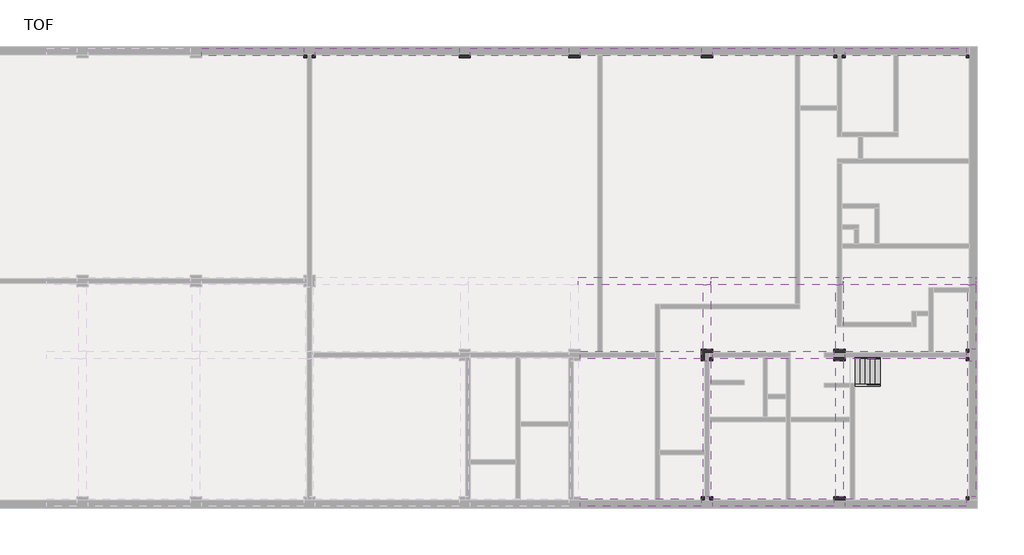
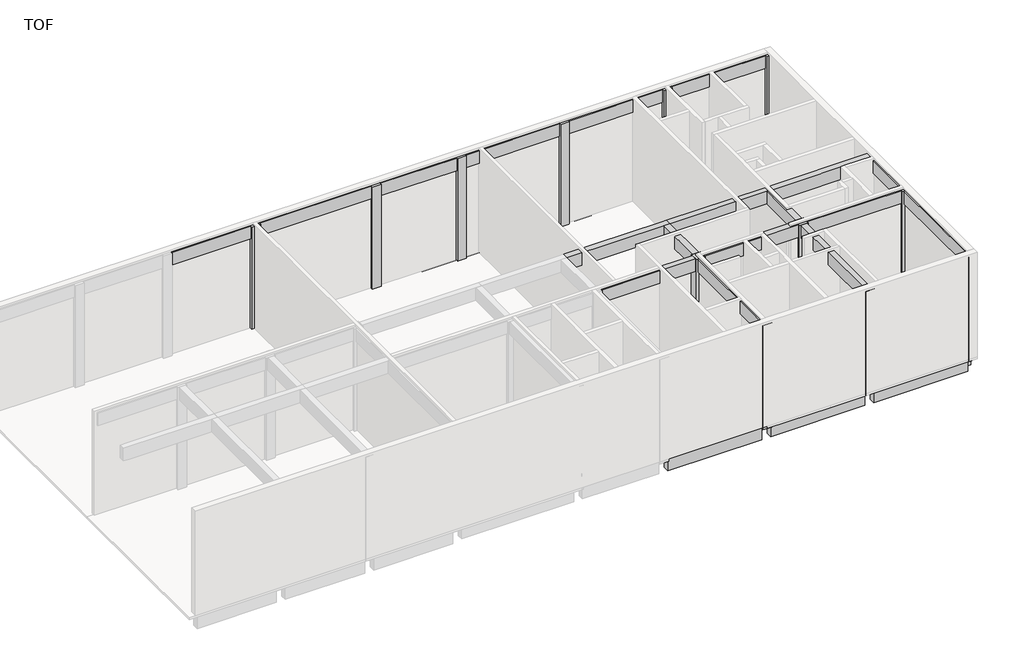
# One storey, part 3 of 3: 32 beams, 12 columns, 2 members, 2 railings, 1 stair flight.
"""IFC4 building model written with IfcOpenShell, lengths in millimetres."""

import ifcopenshell
import ifcopenshell.guid

model = None  # the IFC model being written
_history = None  # IfcOwnerHistory: only IFC2X3 demands one
_inside = {}  # id of a spatial element -> (the spatial element, [elements in it])
_under = {}  # id of a project, library or spatial element -> (it, [spatial elements below it])
_declared = {}  # id of a project -> (the project, [libraries it declares])
_typed = {}  # id of a type object -> (the type object, [elements of that type])
_made_of = {}  # id of a material, layer set ... -> (it, [elements and type objects made of it])


def new_model(schema):
    """Start an empty IFC model of exactly this schema.

    Asked for "IFC4X3", IfcOpenShell would pick the latest addendum, in which some entities
    have other attributes; the version numbers below select the first issue.
    IFC2X3 requires an IfcOwnerHistory on every rooted entity: one is made here for all.
    """
    global model, _history
    if schema == "IFC4X3":
        model = ifcopenshell.file(schema_version=(4, 3, 0, 0))
    else:
        model = ifcopenshell.file(schema=schema)
    _inside.clear()
    _under.clear()
    _declared.clear()
    _typed.clear()
    _made_of.clear()
    _history = None
    if model.schema == "IFC2X3":
        org = make("IfcOrganization", Name="unknown")
        user = make(
            "IfcPersonAndOrganization",
            ThePerson=make("IfcPerson", FamilyName="unknown"),
            TheOrganization=org,
        )
        app = make(
            "IfcApplication",
            ApplicationDeveloper=org,
            Version="unknown",
            ApplicationFullName="unknown",
            ApplicationIdentifier="unknown",
        )
        _history = make(
            "IfcOwnerHistory",
            OwningUser=user,
            OwningApplication=app,
            ChangeAction="ADDED",
            CreationDate=0,
        )
    return model


def make(cls, **values):
    """One entity of the class cls with the attributes given. An attribute that is None is left unset."""
    return model.create_entity(
        cls, **{name: value for name, value in values.items() if value is not None}
    )


def rooted(cls, **values):
    """An entity with a GlobalId (a new one), such as an element, a storey or a relation."""
    return make(cls, GlobalId=ifcopenshell.guid.new(), OwnerHistory=_history, **values)


def si_unit(unit_type, name, prefix=None):
    """IfcSIUnit, for example si_unit("LENGTHUNIT", "METRE", prefix="MILLI")."""
    return make("IfcSIUnit", UnitType=unit_type, Prefix=prefix, Name=name)


def assignment(units):
    """IfcUnitAssignment: the units of a project."""
    return None if units is None else make("IfcUnitAssignment", Units=units)


def point(xyz):
    """IfcCartesianPoint."""
    return None if xyz is None else make("IfcCartesianPoint", Coordinates=xyz)


def direction(xyz):
    """IfcDirection."""
    return None if xyz is None else make("IfcDirection", DirectionRatios=xyz)


def frame(location, z_axis=None, x_axis=None):
    """IfcAxis2Placement3D, a coordinate frame: its origin and axes. An axis left out is left unset."""
    return make(
        "IfcAxis2Placement3D",
        Location=point(location),
        Axis=direction(z_axis),
        RefDirection=direction(x_axis),
    )


def origin():
    """The frame at (0, 0, 0) with its axes left unset."""
    return frame((0.0, 0.0, 0.0))


def place(relative_to, where):
    """IfcLocalPlacement: puts the frame where relative to a parent placement (None: the world)."""
    return make(
        "IfcLocalPlacement", PlacementRelTo=relative_to, RelativePlacement=where
    )


def context(
    kind, dimensions, precision=None, world=None, true_north=None, identifier=None
):
    """IfcGeometricRepresentationContext, for example the 3D "Model" context."""
    return make(
        "IfcGeometricRepresentationContext",
        ContextIdentifier=identifier,
        ContextType=kind,
        CoordinateSpaceDimension=dimensions,
        Precision=precision,
        WorldCoordinateSystem=world,
        TrueNorth=true_north,
    )


def project(units=None, contexts=None):
    """IfcProject with its units and contexts."""
    return rooted(
        "IfcProject",
        Name="project",
        RepresentationContexts=contexts,
        UnitsInContext=assignment(units),
    )


def spatial(cls, under=None, at=None, **own):
    """A site, building, storey or space (cls), placed at a placement, below another one or the project."""
    s = rooted(cls, ObjectPlacement=at, **own)
    if under is not None:
        _under.setdefault(under.id(), (under, []))[1].append(s)
    return s


def polyline(points):
    """IfcPolyline through the points."""
    return make("IfcPolyline", Points=[point(p) for p in points])


def circle_curve(where, radius):
    """IfcCircle in the frame where."""
    return make("IfcCircle", Position=where, Radius=radius)


def ellipse_curve(where, semi_axis1, semi_axis2):
    """IfcEllipse in the frame where."""
    return make(
        "IfcEllipse", Position=where, SemiAxis1=semi_axis1, SemiAxis2=semi_axis2
    )


def outline(outer, holes=None, kind="AREA"):
    """IfcArbitraryClosedProfileDef: a profile drawn as a closed curve; with holes, ...WithVoids."""
    if holes is None:
        return make("IfcArbitraryClosedProfileDef", ProfileType=kind, OuterCurve=outer)
    return make(
        "IfcArbitraryProfileDefWithVoids",
        ProfileType=kind,
        OuterCurve=outer,
        InnerCurves=holes,
    )


def extrude(swept, where, along, depth):
    """IfcExtrudedAreaSolid: the profile swept, set in the frame where, extruded along a direction by depth."""
    return make(
        "IfcExtrudedAreaSolid",
        SweptArea=swept,
        Position=where,
        ExtrudedDirection=direction(along),
        Depth=depth,
    )


def faces_of(points, faces, orient=None, outer=None):
    """IfcFace entities. A face is a list of loops; a loop is a list of indices into points, from 0.

    orient and outer hold one flag for each loop. By default every Orientation is true, the
    first loop of a face is its IfcFaceOuterBound and the others are IfcFaceBound.
    """
    made = []
    for i, loops in enumerate(faces):
        bounds = []
        for j, loop in enumerate(loops):
            is_outer = j == 0 if outer is None else outer[i][j]
            bounds.append(
                make(
                    "IfcFaceOuterBound" if is_outer else "IfcFaceBound",
                    Bound=make("IfcPolyLoop", Polygon=[points[k] for k in loop]),
                    Orientation=True if orient is None else orient[i][j],
                )
            )
        made.append(make("IfcFace", Bounds=bounds))
    return made


def faceted_brep(points, faces, orient=None, outer=None, voids=None):
    """IfcFacetedBrep: a solid bounded by flat faces; with voids (closed shells), ...WithVoids."""
    shared = [point(p) for p in points]
    hull = make("IfcClosedShell", CfsFaces=faces_of(shared, faces, orient, outer))
    if voids is None:
        return make("IfcFacetedBrep", Outer=hull)
    return make(
        "IfcFacetedBrepWithVoids",
        Outer=hull,
        Voids=[
            make(cls, CfsFaces=faces_of(shared, fs, o, b)) for cls, fs, o, b in voids
        ],
    )


def shape(context_of_items, identifier, shape_type, items):
    """IfcShapeRepresentation: the items that make up one representation, for example the "Body"."""
    return make(
        "IfcShapeRepresentation",
        ContextOfItems=context_of_items,
        RepresentationIdentifier=identifier,
        RepresentationType=shape_type,
        Items=items,
    )


def source(mapping_origin, context_of_items, identifier, shape_type, items):
    """IfcRepresentationMap: a shape defined once, which mapped items show again and again."""
    return make(
        "IfcRepresentationMap",
        MappingOrigin=mapping_origin,
        MappedRepresentation=shape(context_of_items, identifier, shape_type, items),
    )


def transform(
    local_origin,
    x_axis=None,
    y_axis=None,
    z_axis=None,
    scale=None,
    scale2=None,
    scale3=None,
    uniform=True,
):
    """IfcCartesianTransformationOperator3D, or its non-uniform kind. x_axis, y_axis, z_axis: its Axis1, 2, 3."""
    if uniform:
        return make(
            "IfcCartesianTransformationOperator3D",
            Axis1=direction(x_axis),
            Axis2=direction(y_axis),
            LocalOrigin=point(local_origin),
            Scale=scale,
            Axis3=direction(z_axis),
        )
    return make(
        "IfcCartesianTransformationOperator3DnonUniform",
        Axis1=direction(x_axis),
        Axis2=direction(y_axis),
        LocalOrigin=point(local_origin),
        Scale=scale,
        Axis3=direction(z_axis),
        Scale2=scale2,
        Scale3=scale3,
    )


def mapped(mapping_source, mapping_target):
    """IfcMappedItem: shows the shape of a source again, moved by a transform."""
    return make(
        "IfcMappedItem", MappingSource=mapping_source, MappingTarget=mapping_target
    )


def made_of(thing, what):
    """Note that an element or type object is made of a material, layer set ...; save() writes the relation."""
    if what is not None:
        _made_of.setdefault(what.id(), (what, []))[1].append(thing)
    return thing


def element(
    cls,
    number,
    at=None,
    inside=None,
    cuts=None,
    type_object=None,
    material=None,
    context=None,
    identifier="Body",
    shape_type=None,
    held_by="IfcProductDefinitionShape",
    body=None,
    shapes=None,
    **own,
):
    """One element of the class cls, such as IfcWall. Its Tag is "e" and its number.

    at: its placement. inside: the storey or other place that contains it. cuts: it is an
    opening in that element (IfcRelVoidsElement). A single representation is given by context,
    identifier, shape_type and body (its items); several are given by shapes. held_by: the class
    of the entity that holds the representations. save() writes the other relations.
    """
    e = rooted(cls, Tag="e%d" % number, ObjectPlacement=at, **own)
    if body is not None:
        shapes = [shape(context, identifier, shape_type, body)]
    if shapes is not None:
        e.Representation = make(held_by, Representations=shapes)
    if inside is not None:
        _inside.setdefault(inside.id(), (inside, []))[1].append(e)
    if cuts is not None:
        rooted(
            "IfcRelVoidsElement", RelatingBuildingElement=cuts, RelatedOpeningElement=e
        )
    if type_object is not None:
        _typed.setdefault(type_object.id(), (type_object, []))[1].append(e)
    return made_of(e, material)


def aggregate(whole, parts):
    """IfcRelAggregates: a whole, such as a stair, and the parts it consists of."""
    return rooted("IfcRelAggregates", RelatingObject=whole, RelatedObjects=parts)


def save(model, path):
    """Write the relations noted so far, then the file.

    IfcRelAggregates (storeys below a building ...), IfcRelContainedInSpatialStructure (elements
    in a storey), IfcRelDefinesByType, IfcRelAssociatesMaterial and IfcRelDeclares: one each for
    every whole, place, type object, material and project.
    """
    for whole, parts in _under.values():
        aggregate(whole, parts)
    for where, things in _inside.values():
        rooted(
            "IfcRelContainedInSpatialStructure",
            RelatedElements=things,
            RelatingStructure=where,
        )
    for kind, things in _typed.values():
        rooted("IfcRelDefinesByType", RelatedObjects=things, RelatingType=kind)
    for what, things in _made_of.values():
        rooted("IfcRelAssociatesMaterial", RelatedObjects=things, RelatingMaterial=what)
    for by, libraries in _declared.values():
        rooted("IfcRelDeclares", RelatingContext=by, RelatedDefinitions=libraries)
    model.write(path)


def plane_surface(at):
    """IfcPlane: the flat surface through the origin of the frame at, square to its z axis."""
    return make("IfcPlane", Position=at)


def cylinder_surface(at, radius):
    """IfcCylindricalSurface: all points at the distance radius from the z axis of the frame at."""
    return make("IfcCylindricalSurface", Position=at, Radius=radius)


def advanced_brep(points, edges, surfaces, faces):
    """IfcAdvancedBrep: a solid bounded by faces that lie on surfaces and meet in shared edges.

    An edge is (start, end): straight between two places in points (the first is 0);
    or (start, end, curve); or (start, end, curve, False) where it runs against its curve.
    A face is (place in surfaces, loops), or (place, loops, False) where it looks against
    its surface's normal. A loop lists edges by number (the first is 1), with a minus sign
    where the edge is run from its end to its start. The first loop is the outer one.
    """
    corners = [point(p) for p in points]
    vertices = [make("IfcVertexPoint", VertexGeometry=c) for c in corners]
    made = []
    for start, end, *more in edges:
        made.append(
            make(
                "IfcEdgeCurve",
                EdgeStart=vertices[start],
                EdgeEnd=vertices[end],
                EdgeGeometry=more[0] if more else make("IfcPolyline", Points=[corners[start], corners[end]]),
                SameSense=more[1] if len(more) > 1 else True,
            )
        )
    hull = []
    for where, loops, *sense in faces:
        bounds = []
        for j, loop in enumerate(loops):
            ring = [make("IfcOrientedEdge", EdgeElement=made[abs(k) - 1], Orientation=k > 0) for k in loop]
            bounds.append(
                make(
                    "IfcFaceOuterBound" if j == 0 else "IfcFaceBound",
                    Bound=make("IfcEdgeLoop", EdgeList=ring),
                    Orientation=True,
                )
            )
        hull.append(make("IfcAdvancedFace", Bounds=bounds, FaceSurface=surfaces[where], SameSense=sense[0] if sense else True))
    return make("IfcAdvancedBrep", Outer=make("IfcClosedShell", CfsFaces=hull))


def railing_36ed9c91(model_context):
    return source(origin(), model_context, "Body", "AdvancedBrep", [
        advanced_brep(
        [(48078.2332408, 8219.6306666, 910.5875748), (48078.2332408, 8249.6306666, 910.5875748), (46993.7216539, 8219.6306666, 1627.8571429), (46993.7216539, 8249.6306666, 1627.8571429), (46728.2332408, 8219.6306666, 1627.8571429), (46728.2332408, 8249.6306666, 1627.8571429)],
        [
            (0, 1, ellipse_curve(frame((48078.2332408, 8234.6306666, 910.5875748), z_axis=(1.0, 0.0, 0.0), x_axis=(0.0, 0.0, -1.0)), 17.9838538, 15.0)),
            (1, 0, ellipse_curve(frame((48078.2332408, 8234.6306666, 910.5875748), z_axis=(1.0, 0.0, 0.0), x_axis=(0.0, 0.0, -1.0)), 17.9838538, 15.0)),
            (0, 2),
            (2, 3, ellipse_curve(frame((46993.7216539, 8234.6306666, 1627.8571429), z_axis=(0.9576224501515418, 0.0, -0.28802646226650325), x_axis=(-0.288026462266502, 0.0, -0.9576224501515423)), 15.6637932, 15.0)),
            (3, 1),
            (3, 2, ellipse_curve(frame((46993.7216539, 8234.6306666, 1627.8571429), z_axis=(0.9576224501515418, 0.0, -0.28802646226650325), x_axis=(-0.288026462266502, 0.0, -0.9576224501515423)), 15.6637932, 15.0)),
            (4, 5, circle_curve(frame((46728.2332408, 8234.6306666, 1627.8571429), z_axis=(-1.0, 0.0, 0.0), x_axis=(0.0, 1.0, 0.0)), 15.0)),
            (5, 4, circle_curve(frame((46728.2332408, 8234.6306666, 1627.8571429), z_axis=(-1.0, 0.0, 0.0), x_axis=(0.0, 1.0, 0.0)), 15.0)),
            (2, 4),
            (5, 3),
        ],
        [
            plane_surface(frame((48078.2332408, 8234.6306666, 928.5714286), z_axis=(1.0, 0.0, 0.0), x_axis=(0.0, -1.0, 0.0))),
            cylinder_surface(frame((48069.9586226, 8234.6306666, 916.0602059), z_axis=(0.8340815140684851, 0.0, -0.5516412130082591), x_axis=(0.0, 1.0, 0.0)), 15.0),
            plane_surface(frame((46728.2332408, 8234.6306666, 1642.8571429), z_axis=(-1.0, 0.0, 0.0), x_axis=(0.0, -1.0, 0.0))),
            cylinder_surface(frame((46998.2332408, 8234.6306666, 1627.8571429), z_axis=(1.0, 0.0, 0.0), x_axis=(0.0, 1.0, 0.0)), 15.0),
        ],
        [
            (0, [[1, 2]]),
            (1, [[-1, 3, 4, 5]]),
            (1, [[-2, -5, 6, -3]]),
            (2, [[7, 8]]),
            (3, [[-4, 9, -8, 10]]),
            (3, [[-6, -10, -7, -9]]),
        ],
    ),
        advanced_brep(
        [(48078.2332408, 8219.6306666, 1410.5875748), (48078.2332408, 8249.6306666, 1410.5875748), (46993.7216539, 8219.6306666, 2127.8571429), (46993.7216539, 8249.6306666, 2127.8571429), (46728.2332408, 8219.6306666, 2127.8571429), (46728.2332408, 8249.6306666, 2127.8571429)],
        [
            (0, 1, ellipse_curve(frame((48078.2332408, 8234.6306666, 1410.5875748), z_axis=(1.0, 0.0, 0.0), x_axis=(0.0, 0.0, -1.0)), 17.9838538, 15.0)),
            (1, 0, ellipse_curve(frame((48078.2332408, 8234.6306666, 1410.5875748), z_axis=(1.0, 0.0, 0.0), x_axis=(0.0, 0.0, -1.0)), 17.9838538, 15.0)),
            (0, 2),
            (2, 3, ellipse_curve(frame((46993.7216539, 8234.6306666, 2127.8571429), z_axis=(0.9576224501515418, 0.0, -0.28802646226650325), x_axis=(-0.288026462266502, 0.0, -0.9576224501515423)), 15.6637932, 15.0)),
            (3, 1),
            (3, 2, ellipse_curve(frame((46993.7216539, 8234.6306666, 2127.8571429), z_axis=(0.9576224501515418, 0.0, -0.28802646226650325), x_axis=(-0.288026462266502, 0.0, -0.9576224501515423)), 15.6637932, 15.0)),
            (4, 5, circle_curve(frame((46728.2332408, 8234.6306666, 2127.8571429), z_axis=(-1.0, 0.0, 0.0), x_axis=(0.0, 1.0, 0.0)), 15.0)),
            (5, 4, circle_curve(frame((46728.2332408, 8234.6306666, 2127.8571429), z_axis=(-1.0, 0.0, 0.0), x_axis=(0.0, 1.0, 0.0)), 15.0)),
            (2, 4),
            (5, 3),
        ],
        [
            plane_surface(frame((48078.2332408, 8234.6306666, 1428.5714286), z_axis=(1.0, 0.0, 0.0), x_axis=(0.0, -1.0, 0.0))),
            cylinder_surface(frame((48069.9586226, 8234.6306666, 1416.0602059), z_axis=(0.8340815140684851, 0.0, -0.5516412130082591), x_axis=(0.0, 1.0, 0.0)), 15.0),
            plane_surface(frame((46728.2332408, 8234.6306666, 2142.8571429), z_axis=(-1.0, 0.0, 0.0), x_axis=(0.0, -1.0, 0.0))),
            cylinder_surface(frame((46998.2332408, 8234.6306666, 2127.8571429), z_axis=(1.0, 0.0, 0.0), x_axis=(0.0, 1.0, 0.0)), 15.0),
        ],
        [
            (0, [[1, 2]]),
            (1, [[-1, 3, 4, 5]]),
            (1, [[-2, -5, 6, -3]]),
            (2, [[7, 8]]),
            (3, [[-4, 9, -8, 10]]),
            (3, [[-6, -10, -7, -9]]),
        ],
    ),
    ])


def railing_d88b3958(model_context):
    return source(origin(), model_context, "Body", "AdvancedBrep", [
        advanced_brep(
        [(48078.2332408, 6875.4306666, 910.5875748), (48078.2332408, 6845.4306666, 910.5875748), (46993.7216539, 6875.4306666, 1627.8571429), (46993.7216539, 6845.4306666, 1627.8571429), (46728.2332408, 6875.4306666, 1627.8571429), (46728.2332408, 6845.4306666, 1627.8571429)],
        [
            (0, 1, ellipse_curve(frame((48078.2332408, 6860.4306666, 910.5875748), z_axis=(1.0, 0.0, 0.0), x_axis=(0.0, 0.0, -1.0)), 17.9838538, 15.0)),
            (1, 0, ellipse_curve(frame((48078.2332408, 6860.4306666, 910.5875748), z_axis=(1.0, 0.0, 0.0), x_axis=(0.0, 0.0, -1.0)), 17.9838538, 15.0)),
            (0, 2),
            (2, 3, ellipse_curve(frame((46993.7216539, 6860.4306666, 1627.8571429), z_axis=(0.9576224501515418, 0.0, -0.28802646226650325), x_axis=(-0.288026462266502, 0.0, -0.9576224501515423)), 15.6637932, 15.0)),
            (3, 1),
            (3, 2, ellipse_curve(frame((46993.7216539, 6860.4306666, 1627.8571429), z_axis=(0.9576224501515418, 0.0, -0.28802646226650325), x_axis=(-0.288026462266502, 0.0, -0.9576224501515423)), 15.6637932, 15.0)),
            (4, 5, circle_curve(frame((46728.2332408, 6860.4306666, 1627.8571429), z_axis=(-1.0, 0.0, 0.0), x_axis=(0.0, -1.0, 0.0)), 15.0)),
            (5, 4, circle_curve(frame((46728.2332408, 6860.4306666, 1627.8571429), z_axis=(-1.0, 0.0, 0.0), x_axis=(0.0, -1.0, 0.0)), 15.0)),
            (2, 4),
            (5, 3),
        ],
        [
            plane_surface(frame((48078.2332408, 6860.4306666, 928.5714286), z_axis=(1.0, 0.0, 0.0), x_axis=(0.0, -1.0, 0.0))),
            cylinder_surface(frame((48069.9586226, 6860.4306666, 916.0602059), z_axis=(0.8340815140684851, 0.0, -0.5516412130082591), x_axis=(0.0, -1.0, 0.0)), 15.0),
            plane_surface(frame((46728.2332408, 6860.4306666, 1642.8571429), z_axis=(-1.0, 0.0, 0.0), x_axis=(0.0, -1.0, 0.0))),
            cylinder_surface(frame((46998.2332408, 6860.4306666, 1627.8571429), z_axis=(1.0, 0.0, 0.0), x_axis=(0.0, -1.0, 0.0)), 15.0),
        ],
        [
            (0, [[1, 2]]),
            (1, [[-1, 3, 4, 5]]),
            (1, [[-2, -5, 6, -3]]),
            (2, [[7, 8]]),
            (3, [[-4, 9, -8, 10]]),
            (3, [[-6, -10, -7, -9]]),
        ],
    ),
        advanced_brep(
        [(48078.2332408, 6875.4306666, 1410.5875748), (48078.2332408, 6845.4306666, 1410.5875748), (46993.7216539, 6875.4306666, 2127.8571429), (46993.7216539, 6845.4306666, 2127.8571429), (46728.2332408, 6875.4306666, 2127.8571429), (46728.2332408, 6845.4306666, 2127.8571429)],
        [
            (0, 1, ellipse_curve(frame((48078.2332408, 6860.4306666, 1410.5875748), z_axis=(1.0, 0.0, 0.0), x_axis=(0.0, 0.0, -1.0)), 17.9838538, 15.0)),
            (1, 0, ellipse_curve(frame((48078.2332408, 6860.4306666, 1410.5875748), z_axis=(1.0, 0.0, 0.0), x_axis=(0.0, 0.0, -1.0)), 17.9838538, 15.0)),
            (0, 2),
            (2, 3, ellipse_curve(frame((46993.7216539, 6860.4306666, 2127.8571429), z_axis=(0.9576224501515418, 0.0, -0.28802646226650325), x_axis=(-0.288026462266502, 0.0, -0.9576224501515423)), 15.6637932, 15.0)),
            (3, 1),
            (3, 2, ellipse_curve(frame((46993.7216539, 6860.4306666, 2127.8571429), z_axis=(0.9576224501515418, 0.0, -0.28802646226650325), x_axis=(-0.288026462266502, 0.0, -0.9576224501515423)), 15.6637932, 15.0)),
            (4, 5, circle_curve(frame((46728.2332408, 6860.4306666, 2127.8571429), z_axis=(-1.0, 0.0, 0.0), x_axis=(0.0, -1.0, 0.0)), 15.0)),
            (5, 4, circle_curve(frame((46728.2332408, 6860.4306666, 2127.8571429), z_axis=(-1.0, 0.0, 0.0), x_axis=(0.0, -1.0, 0.0)), 15.0)),
            (2, 4),
            (5, 3),
        ],
        [
            plane_surface(frame((48078.2332408, 6860.4306666, 1428.5714286), z_axis=(1.0, 0.0, 0.0), x_axis=(0.0, -1.0, 0.0))),
            cylinder_surface(frame((48069.9586226, 6860.4306666, 1416.0602059), z_axis=(0.8340815140684851, 0.0, -0.5516412130082591), x_axis=(0.0, -1.0, 0.0)), 15.0),
            plane_surface(frame((46728.2332408, 6860.4306666, 2142.8571429), z_axis=(-1.0, 0.0, 0.0), x_axis=(0.0, -1.0, 0.0))),
            cylinder_surface(frame((46998.2332408, 6860.4306666, 2127.8571429), z_axis=(1.0, 0.0, 0.0), x_axis=(0.0, -1.0, 0.0)), 15.0),
        ],
        [
            (0, [[1, 2]]),
            (1, [[-1, 3, 4, 5]]),
            (1, [[-2, -5, 6, -3]]),
            (2, [[7, 8]]),
            (3, [[-4, 9, -8, 10]]),
            (3, [[-6, -10, -7, -9]]),
        ],
    ),
    ])


def stair_flight_4e27faa5(model_context):
    return source(origin(), model_context, "Body", "SweptSolid", [
        extrude(outline(polyline([(47808.2332408, 6860.0306666), (47808.2332408, 8235.0306666), (48078.2332408, 8235.0306666), (48078.2332408, 6860.0306666), (47808.2332408, 6860.0306666)])), frame((0.0, 0.0, 296.5714286), z_axis=(0.0, 0.0, 1.0), x_axis=(1.0, 0.0, 0.0)), (0.0, 0.0, 1.0), 32.0),
        extrude(outline(polyline([(47538.2332408, 6860.0306666), (47538.2332408, 8235.0306666), (47808.2332408, 8235.0306666), (47808.2332408, 6860.0306666), (47538.2332408, 6860.0306666)])), frame((0.0, 0.0, 475.1428571), z_axis=(0.0, 0.0, 1.0), x_axis=(1.0, 0.0, 0.0)), (0.0, 0.0, 1.0), 32.0),
        extrude(outline(polyline([(47268.2332408, 6860.0306666), (47268.2332408, 8235.0306666), (47538.2332408, 8235.0306666), (47538.2332408, 6860.0306666), (47268.2332408, 6860.0306666)])), frame((0.0, 0.0, 653.7142857), z_axis=(0.0, 0.0, 1.0), x_axis=(1.0, 0.0, 0.0)), (0.0, 0.0, 1.0), 32.0),
        extrude(outline(polyline([(46998.2332408, 6860.0306666), (46998.2332408, 8235.0306666), (47268.2332408, 8235.0306666), (47268.2332408, 6860.0306666), (46998.2332408, 6860.0306666)])), frame((0.0, 0.0, 832.2857143), z_axis=(0.0, 0.0, 1.0), x_axis=(1.0, 0.0, 0.0)), (0.0, 0.0, 1.0), 32.0),
        extrude(outline(polyline([(46728.2332408, 6860.0306666), (46728.2332408, 8235.0306666), (46998.2332408, 8235.0306666), (46998.2332408, 6860.0306666), (46728.2332408, 6860.0306666)])), frame((0.0, 0.0, 1010.8571429), z_axis=(0.0, 0.0, 1.0), x_axis=(1.0, 0.0, 0.0)), (0.0, 0.0, 1.0), 32.0),
    ])


model = new_model("IFC4")

# Units and contexts
model_context = context("Model", 3, world=origin())
ifc_project = project(units=[si_unit("LENGTHUNIT", "METRE", prefix="MILLI")], contexts=[model_context])

# Site, building, storey
site = spatial("IfcSite", under=ifc_project)
building = spatial("IfcBuilding", under=site)
storey = spatial("IfcBuildingStorey", under=building, Name="TOF", Elevation=150.0)

# Beams
placement = place(None, origin())
element("IfcBeam", 1, ObjectType="RC Beam_Rectangular", at=placement, inside=storey, context=model_context, shape_type="SweptSolid", body=[
    extrude(outline(polyline([(52724.7, 24116.5208589), (53124.7, 24116.5208589), (53124.7, 18966.5208589), (52724.7, 18966.5208589), (52724.7, 24116.5208589)])), frame((0.0, 0.0, -750.0), z_axis=(0.0, 0.0, 1.0), x_axis=(1.0, 0.0, 0.0)), (0.0, 0.0, 1.0), 900.0),
    extrude(outline(polyline([(53124.7, 8716.5208589), (52724.7, 8716.5208589), (52724.7, 18366.5208589), (53124.7, 18366.5208589), (53124.7, 8716.5208589)])), frame((0.0, 0.0, -750.0), z_axis=(0.0, 0.0, 1.0), x_axis=(1.0, 0.0, 0.0)), (0.0, 0.0, 1.0), 900.0),
])
element("IfcBeam", 2, ObjectType="RC Beam_Rectangular", at=placement, inside=storey, context=model_context, shape_type="SweptSolid", body=[
    extrude(outline(polyline([(52724.7, 8116.5208589), (53124.7, 8116.5208589), (53124.7, 916.5208589), (52724.7, 916.5208589), (52724.7, 8116.5208589)])), frame((0.0, 0.0, -750.0), z_axis=(0.0, 0.0, 1.0), x_axis=(1.0, 0.0, 0.0)), (0.0, 0.0, 1.0), 900.0),
])
element("IfcBeam", 3, ObjectType="RC Beam_Rectangular", at=placement, inside=storey, context=model_context, shape_type="SweptSolid", body=[
    extrude(outline(polyline([(12224.7, 24216.5208589), (12224.7, 24616.5208589), (17624.7, 24616.5208589), (17624.7, 24216.5208589), (12224.7, 24216.5208589)])), frame((0.0, 0.0, -900.0), z_axis=(0.0, 0.0, 1.0), x_axis=(1.0, 0.0, 0.0)), (0.0, 0.0, 1.0), 900.0),
])
element("IfcBeam", 4, ObjectType="RC Beam_Rectangular", at=placement, inside=storey, context=model_context, shape_type="SweptSolid", body=[
    extrude(outline(polyline([(18224.7, 24216.5208589), (18224.7, 24616.5208589), (25824.7, 24616.5208589), (25824.7, 24216.5208589), (18224.7, 24216.5208589)])), frame((0.0, 0.0, -750.0), z_axis=(0.0, 0.0, 1.0), x_axis=(1.0, 0.0, 0.0)), (0.0, 0.0, 1.0), 900.0),
])
element("IfcBeam", 5, ObjectType="RC Beam_Rectangular", at=placement, inside=storey, context=model_context, shape_type="SweptSolid", body=[
    extrude(outline(polyline([(26424.7, 24216.5208589), (26424.7, 24616.5208589), (31624.7, 24616.5208589), (31624.7, 24216.5208589), (26424.7, 24216.5208589)])), frame((0.0, 0.0, -750.0), z_axis=(0.0, 0.0, 1.0), x_axis=(1.0, 0.0, 0.0)), (0.0, 0.0, 1.0), 900.0),
])
element("IfcBeam", 6, ObjectType="RC Beam_Rectangular", at=placement, inside=storey, context=model_context, shape_type="SweptSolid", body=[
    extrude(outline(polyline([(32224.7, 24216.5208589), (32224.7, 24616.5208589), (38624.7, 24616.5208589), (38624.7, 24216.5208589), (32224.7, 24216.5208589)])), frame((0.0, 0.0, -750.0), z_axis=(0.0, 0.0, 1.0), x_axis=(1.0, 0.0, 0.0)), (0.0, 0.0, 1.0), 900.0),
])
element("IfcBeam", 7, ObjectType="RC Beam_Rectangular", at=placement, inside=storey, context=model_context, shape_type="SweptSolid", body=[
    extrude(outline(polyline([(39224.7, 24216.5208589), (39224.7, 24616.5208589), (45624.7, 24616.5208589), (45624.7, 24216.5208589), (39224.7, 24216.5208589)])), frame((0.0, 0.0, -750.0), z_axis=(0.0, 0.0, 1.0), x_axis=(1.0, 0.0, 0.0)), (0.0, 0.0, 1.0), 900.0),
])
element("IfcBeam", 8, ObjectType="RC Beam_Rectangular", at=placement, inside=storey, context=model_context, shape_type="SweptSolid", body=[
    extrude(outline(polyline([(46224.7, 24216.5208589), (46224.7, 24616.5208589), (52624.7, 24616.5208589), (52624.7, 24216.5208589), (46224.7, 24216.5208589)])), frame((0.0, 0.0, -750.0), z_axis=(0.0, 0.0, 1.0), x_axis=(1.0, 0.0, 0.0)), (0.0, 0.0, 1.0), 900.0),
])
element("IfcBeam", 9, ObjectType="RC Beam_Rectangular", at=placement, inside=storey, context=model_context, shape_type="SweptSolid", body=[
    extrude(outline(polyline([(32224.7, 416.5208589), (32224.7, 816.5208589), (38624.7, 816.5208589), (38624.7, 416.5208589), (32224.7, 416.5208589)])), frame((0.0, 0.0, -750.0), z_axis=(0.0, 0.0, 1.0), x_axis=(1.0, 0.0, 0.0)), (0.0, 0.0, 1.0), 900.0),
])
element("IfcBeam", 10, ObjectType="RC Beam_Rectangular", at=placement, inside=storey, context=model_context, shape_type="SweptSolid", body=[
    extrude(outline(polyline([(39224.7, 416.5208589), (39224.7, 816.5208589), (45624.7, 816.5208589), (45624.7, 416.5208589), (39224.7, 416.5208589)])), frame((0.0, 0.0, -750.0), z_axis=(0.0, 0.0, 1.0), x_axis=(1.0, 0.0, 0.0)), (0.0, 0.0, 1.0), 900.0),
])
element("IfcBeam", 11, ObjectType="RC Beam_Rectangular", at=placement, inside=storey, context=model_context, shape_type="SweptSolid", body=[
    extrude(outline(polyline([(46224.7, 416.5208589), (46224.7, 816.5208589), (52624.7, 816.5208589), (52624.7, 416.5208589), (46224.7, 416.5208589)])), frame((0.0, 0.0, -750.0), z_axis=(0.0, 0.0, 1.0), x_axis=(1.0, 0.0, 0.0)), (0.0, 0.0, 1.0), 900.0),
])
element("IfcBeam", 12, ObjectType="RC Beam_Rectangular", at=placement, inside=storey, context=model_context, shape_type="Brep", body=[
    faceted_brep([(39124.7, 12116.5208589, 7500.0), (39124.7, 12303.8208589, 7500.0), (39124.7, 12516.5208589, 7500.0), (38724.7, 12516.5208589, 7500.0), (32124.7, 12516.5208589, 7500.0), (32124.7, 12116.5208589, 7500.0), (38724.7, 12116.5208589, 7500.0), (39124.7, 12116.5208589, 6600.0), (32124.7, 12116.5208589, 6600.0), (38724.7, 12116.5208589, 6600.0), (39124.7, 12516.5208589, 6600.0), (32124.7, 12516.5208589, 6600.0), (39124.7, 12516.5208589, 6750.0)], [[[0, 1, 2, 3, 4, 5, 6]], [[7, 0, 6, 5, 8, 9]], [[10, 7, 9, 8, 11]], [[2, 12, 10, 11, 4, 3]], [[2, 1, 0, 7, 10, 12]], [[5, 4, 11, 8]]]),
])
element("IfcBeam", 13, ObjectType="RC Beam_Rectangular", at=placement, inside=storey, context=model_context, shape_type="Brep", body=[
    faceted_brep([(46124.7, 12116.5208589, 7500.0), (46124.7, 12303.8208589, 7500.0), (46124.7, 12516.5208589, 7500.0), (45724.7, 12516.5208589, 7500.0), (39124.7, 12516.5208589, 7500.0), (39124.7, 12116.5208589, 7500.0), (45724.7, 12116.5208589, 7500.0), (46124.7, 12116.5208589, 6600.0), (39124.7, 12116.5208589, 6600.0), (45724.7, 12116.5208589, 6600.0), (46124.7, 12516.5208589, 6600.0), (39124.7, 12516.5208589, 6600.0), (46124.7, 12516.5208589, 6750.0)], [[[0, 1, 2, 3, 4, 5, 6]], [[7, 0, 6, 5, 8, 9]], [[10, 7, 9, 8, 11]], [[2, 12, 10, 11, 4, 3]], [[2, 1, 0, 7, 10, 12]], [[5, 4, 11, 8]]]),
])
element("IfcBeam", 14, ObjectType="RC Beam_Rectangular", at=placement, inside=storey, context=model_context, shape_type="Brep", body=[
    faceted_brep([(53124.7, 12116.5208589, 7500.0), (53124.7, 12303.8208589, 7500.0), (53124.7, 12516.5208589, 7500.0), (52724.7, 12516.5208589, 7500.0), (46124.7, 12516.5208589, 7500.0), (46124.7, 12116.5208589, 7500.0), (52724.7, 12116.5208589, 7500.0), (53124.7, 12116.5208589, 6600.0), (46124.7, 12116.5208589, 6600.0), (52724.7, 12116.5208589, 6600.0), (53124.7, 12516.5208589, 6600.0), (46124.7, 12516.5208589, 6600.0), (53124.7, 12516.5208589, 6750.0)], [[[0, 1, 2, 3, 4, 5, 6]], [[7, 0, 6, 5, 8, 9]], [[10, 7, 9, 8, 11]], [[2, 12, 10, 11, 4, 3]], [[2, 1, 0, 7, 10, 12]], [[5, 4, 11, 8]]]),
])
element("IfcBeam", 15, ObjectType="RC Beam_Rectangular", at=placement, inside=storey, context=model_context, shape_type="SweptSolid", body=[
    extrude(outline(polyline([(12224.7, 24216.5208589), (12224.7, 24616.5208589), (17624.7, 24616.5208589), (17624.7, 24216.5208589), (12224.7, 24216.5208589)])), frame((0.0, 0.0, 6600.0), z_axis=(0.0, 0.0, 1.0), x_axis=(1.0, 0.0, 0.0)), (0.0, 0.0, 1.0), 900.0),
])
element("IfcBeam", 16, ObjectType="RC Beam_Rectangular", at=placement, inside=storey, context=model_context, shape_type="SweptSolid", body=[
    extrude(outline(polyline([(18224.7, 24216.5208589), (18224.7, 24616.5208589), (25824.7, 24616.5208589), (25824.7, 24216.5208589), (18224.7, 24216.5208589)])), frame((0.0, 0.0, 6600.0), z_axis=(0.0, 0.0, 1.0), x_axis=(1.0, 0.0, 0.0)), (0.0, 0.0, 1.0), 900.0),
])
element("IfcBeam", 17, ObjectType="RC Beam_Rectangular", at=placement, inside=storey, context=model_context, shape_type="SweptSolid", body=[
    extrude(outline(polyline([(26424.7, 24216.5208589), (26424.7, 24616.5208589), (31624.7, 24616.5208589), (31624.7, 24216.5208589), (26424.7, 24216.5208589)])), frame((0.0, 0.0, 6600.0), z_axis=(0.0, 0.0, 1.0), x_axis=(1.0, 0.0, 0.0)), (0.0, 0.0, 1.0), 900.0),
])
element("IfcBeam", 18, ObjectType="RC Beam_Rectangular", at=placement, inside=storey, context=model_context, shape_type="SweptSolid", body=[
    extrude(outline(polyline([(32224.7, 24216.5208589), (32224.7, 24616.5208589), (38624.7, 24616.5208589), (38624.7, 24216.5208589), (32224.7, 24216.5208589)])), frame((0.0, 0.0, 6600.0), z_axis=(0.0, 0.0, 1.0), x_axis=(1.0, 0.0, 0.0)), (0.0, 0.0, 1.0), 900.0),
])
element("IfcBeam", 19, ObjectType="RC Beam_Rectangular", at=placement, inside=storey, context=model_context, shape_type="SweptSolid", body=[
    extrude(outline(polyline([(39224.7, 24216.5208589), (39224.7, 24616.5208589), (45624.7, 24616.5208589), (45624.7, 24216.5208589), (39224.7, 24216.5208589)])), frame((0.0, 0.0, 6600.0), z_axis=(0.0, 0.0, 1.0), x_axis=(1.0, 0.0, 0.0)), (0.0, 0.0, 1.0), 900.0),
])
element("IfcBeam", 20, ObjectType="RC Beam_Rectangular", at=placement, inside=storey, context=model_context, shape_type="SweptSolid", body=[
    extrude(outline(polyline([(46224.7, 24216.5208589), (46224.7, 24616.5208589), (52624.7, 24616.5208589), (52624.7, 24216.5208589), (46224.7, 24216.5208589)])), frame((0.0, 0.0, 6600.0), z_axis=(0.0, 0.0, 1.0), x_axis=(1.0, 0.0, 0.0)), (0.0, 0.0, 1.0), 900.0),
])
element("IfcBeam", 21, ObjectType="RC Beam_Rectangular", at=placement, inside=storey, context=model_context, shape_type="SweptSolid", body=[
    extrude(outline(polyline([(32224.7, 8216.5208589), (32224.7, 8616.5208589), (38624.7, 8616.5208589), (38624.7, 8216.5208589), (32224.7, 8216.5208589)])), frame((0.0, 0.0, 6600.0), z_axis=(0.0, 0.0, 1.0), x_axis=(1.0, 0.0, 0.0)), (0.0, 0.0, 1.0), 900.0),
])
element("IfcBeam", 22, ObjectType="RC Beam_Rectangular", at=placement, inside=storey, context=model_context, shape_type="SweptSolid", body=[
    extrude(outline(polyline([(39224.7, 8216.5208589), (39224.7, 8616.5208589), (45624.7, 8616.5208589), (45624.7, 8216.5208589), (39224.7, 8216.5208589)])), frame((0.0, 0.0, 6600.0), z_axis=(0.0, 0.0, 1.0), x_axis=(1.0, 0.0, 0.0)), (0.0, 0.0, 1.0), 900.0),
])
element("IfcBeam", 23, ObjectType="RC Beam_Rectangular", at=placement, inside=storey, context=model_context, shape_type="SweptSolid", body=[
    extrude(outline(polyline([(46224.7, 8216.5208589), (46224.7, 8616.5208589), (52624.7, 8616.5208589), (52624.7, 8216.5208589), (46224.7, 8216.5208589)])), frame((0.0, 0.0, 6600.0), z_axis=(0.0, 0.0, 1.0), x_axis=(1.0, 0.0, 0.0)), (0.0, 0.0, 1.0), 900.0),
])
element("IfcBeam", 24, ObjectType="RC Beam_Rectangular", at=placement, inside=storey, context=model_context, shape_type="SweptSolid", body=[
    extrude(outline(polyline([(32224.7, 416.5208589), (32224.7, 816.5208589), (38624.7, 816.5208589), (38624.7, 416.5208589), (32224.7, 416.5208589)])), frame((0.0, 0.0, 6600.0), z_axis=(0.0, 0.0, 1.0), x_axis=(1.0, 0.0, 0.0)), (0.0, 0.0, 1.0), 900.0),
])
element("IfcBeam", 25, ObjectType="RC Beam_Rectangular", at=placement, inside=storey, context=model_context, shape_type="SweptSolid", body=[
    extrude(outline(polyline([(39224.7, 416.5208589), (39224.7, 816.5208589), (45624.7, 816.5208589), (45624.7, 416.5208589), (39224.7, 416.5208589)])), frame((0.0, 0.0, 6600.0), z_axis=(0.0, 0.0, 1.0), x_axis=(1.0, 0.0, 0.0)), (0.0, 0.0, 1.0), 900.0),
])
element("IfcBeam", 26, ObjectType="RC Beam_Rectangular", at=placement, inside=storey, context=model_context, shape_type="SweptSolid", body=[
    extrude(outline(polyline([(46224.7, 416.5208589), (46224.7, 816.5208589), (52624.7, 816.5208589), (52624.7, 416.5208589), (46224.7, 416.5208589)])), frame((0.0, 0.0, 6600.0), z_axis=(0.0, 0.0, 1.0), x_axis=(1.0, 0.0, 0.0)), (0.0, 0.0, 1.0), 900.0),
])
element("IfcBeam", 27, ObjectType="RC Beam_Rectangular", at=placement, inside=storey, context=model_context, shape_type="SweptSolid", body=[
    extrude(outline(polyline([(38724.7, 8116.5208589), (39124.7, 8116.5208589), (39124.7, 916.5208589), (38724.7, 916.5208589), (38724.7, 8116.5208589)])), frame((0.0, 0.0, 6600.0), z_axis=(0.0, 0.0, 1.0), x_axis=(1.0, 0.0, 0.0)), (0.0, 0.0, 1.0), 900.0),
])
element("IfcBeam", 28, ObjectType="RC Beam_Rectangular", at=placement, inside=storey, context=model_context, shape_type="SweptSolid", body=[
    extrude(outline(polyline([(38724.7, 12116.5208589), (39124.7, 12116.5208589), (39124.7, 8716.5208589), (38724.7, 8716.5208589), (38724.7, 12116.5208589)])), frame((0.0, 0.0, 6600.0), z_axis=(0.0, 0.0, 1.0), x_axis=(1.0, 0.0, 0.0)), (0.0, 0.0, 1.0), 900.0),
])
element("IfcBeam", 29, ObjectType="RC Beam_Rectangular", at=placement, inside=storey, context=model_context, shape_type="SweptSolid", body=[
    extrude(outline(polyline([(45724.7, 8116.5208589), (46124.7, 8116.5208589), (46124.7, 916.5208589), (45724.7, 916.5208589), (45724.7, 8116.5208589)])), frame((0.0, 0.0, 6600.0), z_axis=(0.0, 0.0, 1.0), x_axis=(1.0, 0.0, 0.0)), (0.0, 0.0, 1.0), 900.0),
])
element("IfcBeam", 30, ObjectType="RC Beam_Rectangular", at=placement, inside=storey, context=model_context, shape_type="SweptSolid", body=[
    extrude(outline(polyline([(45724.7, 12116.5208589), (46124.7, 12116.5208589), (46124.7, 8716.5208589), (45724.7, 8716.5208589), (45724.7, 12116.5208589)])), frame((0.0, 0.0, 6600.0), z_axis=(0.0, 0.0, 1.0), x_axis=(1.0, 0.0, 0.0)), (0.0, 0.0, 1.0), 900.0),
])
element("IfcBeam", 31, ObjectType="RC Beam_Rectangular", at=placement, inside=storey, context=model_context, shape_type="SweptSolid", body=[
    extrude(outline(polyline([(52724.7, 8116.5208589), (53124.7, 8116.5208589), (53124.7, 916.5208589), (52724.7, 916.5208589), (52724.7, 8116.5208589)])), frame((0.0, 0.0, 6600.0), z_axis=(0.0, 0.0, 1.0), x_axis=(1.0, 0.0, 0.0)), (0.0, 0.0, 1.0), 900.0),
])
element("IfcBeam", 32, ObjectType="RC Beam_Rectangular", at=placement, inside=storey, context=model_context, shape_type="SweptSolid", body=[
    extrude(outline(polyline([(52724.7, 12116.5208589), (53124.7, 12116.5208589), (53124.7, 8716.5208589), (52724.7, 8716.5208589), (52724.7, 12116.5208589)])), frame((0.0, 0.0, 6600.0), z_axis=(0.0, 0.0, 1.0), x_axis=(1.0, 0.0, 0.0)), (0.0, 0.0, 1.0), 900.0),
])

# Columns
element("IfcColumn", 33, ObjectType="RC_Column_Rectangular", at=placement, inside=storey, context=model_context, shape_type="Brep", body=[
    faceted_brep([(18224.7, 24716.5208589, 7500.0), (18224.7, 24616.5208589, 7500.0), (18224.7, 24216.5208589, 7500.0), (18224.7, 24116.5208589, 7500.0), (18224.7, 24116.5208589, 150.0), (18224.7, 24716.5208589, 150.0), (18124.7, 24116.5208589, 7500.0), (17724.7, 24116.5208589, 7500.0), (17624.7, 24116.5208589, 7500.0), (17624.7, 24116.5208589, 150.0), (17624.7, 24216.5208589, 7500.0), (17624.7, 24616.5208589, 7500.0), (17624.7, 24716.5208589, 7500.0), (17624.7, 24716.5208589, 150.0)], [[[0, 1, 2, 3, 4, 5]], [[3, 6, 7, 8, 9, 4]], [[8, 10, 11, 12, 13, 9]], [[12, 0, 5, 13]], [[3, 2, 1, 0, 12, 11, 10, 8, 7, 6]], [[5, 4, 9, 13]]]),
])
element("IfcColumn", 34, ObjectType="RC_Column_Rectangular", at=placement, inside=storey, context=model_context, shape_type="Brep", body=[
    faceted_brep([(26424.7, 24716.5208589, 7500.0), (26424.7, 24616.5208589, 7500.0), (26424.7, 24216.5208589, 7500.0), (26424.7, 24116.5208589, 7500.0), (26424.7, 24116.5208589, 150.0), (26424.7, 24716.5208589, 150.0), (26324.7, 24116.5208589, 7500.0), (25924.7, 24116.5208589, 7500.0), (25824.7, 24116.5208589, 7500.0), (25824.7, 24116.5208589, 150.0), (25824.7, 24216.5208589, 7500.0), (25824.7, 24616.5208589, 7500.0), (25824.7, 24716.5208589, 7500.0), (25824.7, 24716.5208589, 150.0)], [[[0, 1, 2, 3, 4, 5]], [[3, 6, 7, 8, 9, 4]], [[8, 10, 11, 12, 13, 9]], [[12, 0, 5, 13]], [[3, 2, 1, 0, 12, 11, 10, 8, 7, 6]], [[5, 4, 9, 13]]]),
])
element("IfcColumn", 35, ObjectType="RC_Column_Rectangular", at=placement, inside=storey, context=model_context, shape_type="Brep", body=[
    faceted_brep([(32224.7, 24716.5208589, 7500.0), (32224.7, 24616.5208589, 7500.0), (32224.7, 24216.5208589, 7500.0), (32224.7, 24116.5208589, 7500.0), (32224.7, 24116.5208589, 150.0), (32224.7, 24716.5208589, 150.0), (32124.7, 24116.5208589, 7500.0), (31724.7, 24116.5208589, 7500.0), (31624.7, 24116.5208589, 7500.0), (31624.7, 24116.5208589, 150.0), (31624.7, 24216.5208589, 7500.0), (31624.7, 24616.5208589, 7500.0), (31624.7, 24716.5208589, 7500.0), (31624.7, 24716.5208589, 150.0)], [[[0, 1, 2, 3, 4, 5]], [[3, 6, 7, 8, 9, 4]], [[8, 10, 11, 12, 13, 9]], [[12, 0, 5, 13]], [[3, 2, 1, 0, 12, 11, 10, 8, 7, 6]], [[5, 4, 9, 13]]]),
])
element("IfcColumn", 36, ObjectType="RC_Column_Rectangular", at=placement, inside=storey, context=model_context, shape_type="Brep", body=[
    faceted_brep([(39224.7, 24716.5208589, 7500.0), (39224.7, 24616.5208589, 7500.0), (39224.7, 24216.5208589, 7500.0), (39224.7, 24116.5208589, 7500.0), (39224.7, 24116.5208589, 150.0), (39224.7, 24716.5208589, 150.0), (39124.7, 24116.5208589, 7500.0), (38724.7, 24116.5208589, 7500.0), (38624.7, 24116.5208589, 7500.0), (38624.7, 24116.5208589, 150.0), (38624.7, 24216.5208589, 7500.0), (38624.7, 24616.5208589, 7500.0), (38624.7, 24716.5208589, 7500.0), (38624.7, 24716.5208589, 150.0)], [[[0, 1, 2, 3, 4, 5]], [[3, 6, 7, 8, 9, 4]], [[8, 10, 11, 12, 13, 9]], [[12, 0, 5, 13]], [[3, 2, 1, 0, 12, 11, 10, 8, 7, 6]], [[5, 4, 9, 13]]]),
])
element("IfcColumn", 37, ObjectType="RC_Column_Rectangular", at=placement, inside=storey, context=model_context, shape_type="Brep", body=[
    faceted_brep([(46224.7, 24716.5208589, 0.0), (46224.7, 24116.5208589, 0.0), (45624.7, 24116.5208589, 0.0), (45624.7, 24716.5208589, 0.0), (46224.7, 24716.5208589, 7500.0), (46224.7, 24616.5208589, 7500.0), (46224.7, 24216.5208589, 7500.0), (46224.7, 24116.5208589, 7500.0), (46124.7, 24116.5208589, 7500.0), (45724.7, 24116.5208589, 7500.0), (45624.7, 24116.5208589, 7500.0), (45624.7, 24216.5208589, 7500.0), (45624.7, 24616.5208589, 7500.0), (45624.7, 24716.5208589, 7500.0)], [[[0, 1, 2, 3]], [[4, 5, 6, 7, 1, 0]], [[7, 8, 9, 10, 2, 1]], [[10, 11, 12, 13, 3, 2]], [[13, 4, 0, 3]], [[4, 13, 12, 11, 10, 9, 8, 7, 6, 5]]]),
])
element("IfcColumn", 38, ObjectType="RC_Column_Rectangular", at=placement, inside=storey, context=model_context, shape_type="Brep", body=[
    faceted_brep([(53224.7, 24716.5208589, 0.0), (53224.7, 24116.5208589, 0.0), (52624.7, 24116.5208589, 0.0), (52624.7, 24716.5208589, 0.0), (53224.7, 24716.5208589, 7500.0), (53224.7, 24116.5208589, 7500.0), (53124.7, 24116.5208589, 7500.0), (52724.7, 24116.5208589, 7500.0), (52624.7, 24116.5208589, 7500.0), (52624.7, 24216.5208589, 7500.0), (52624.7, 24616.5208589, 7500.0), (52624.7, 24716.5208589, 7500.0)], [[[0, 1, 2, 3]], [[4, 5, 1, 0]], [[5, 6, 7, 8, 2, 1]], [[8, 9, 10, 11, 3, 2]], [[11, 4, 0, 3]], [[4, 11, 10, 9, 8, 7, 6, 5]]]),
])
element("IfcColumn", 39, ObjectType="RC_Column_Rectangular", at=placement, inside=storey, context=model_context, shape_type="Brep", body=[
    faceted_brep([(39224.7, 8716.5208589, 0.0), (39224.7, 8116.5208589, 0.0), (38624.7, 8116.5208589, 0.0), (38624.7, 8716.5208589, 0.0), (39224.7, 8716.5208589, 7500.0), (39224.7, 8616.5208589, 7500.0), (39224.7, 8216.5208589, 7500.0), (39224.7, 8116.5208589, 7500.0), (39124.7, 8116.5208589, 7500.0), (38724.7, 8116.5208589, 7500.0), (38624.7, 8116.5208589, 7500.0), (38624.7, 8216.5208589, 7500.0), (38624.7, 8616.5208589, 7500.0), (38624.7, 8716.5208589, 7500.0), (38724.7, 8716.5208589, 7500.0), (39124.7, 8716.5208589, 7500.0)], [[[0, 1, 2, 3]], [[1, 0, 4, 5, 6, 7]], [[2, 1, 7, 8, 9, 10]], [[3, 2, 10, 11, 12, 13]], [[0, 3, 13, 14, 15, 4]], [[7, 6, 5, 4, 15, 14, 13, 12, 11, 10, 9, 8]]]),
])
element("IfcColumn", 40, ObjectType="RC_Column_Rectangular", at=placement, inside=storey, context=model_context, shape_type="Brep", body=[
    faceted_brep([(46224.7, 8716.5208589, 0.0), (46224.7, 8116.5208589, 0.0), (45624.7, 8116.5208589, 0.0), (45624.7, 8716.5208589, 0.0), (46224.7, 8716.5208589, 7500.0), (46224.7, 8616.5208589, 7500.0), (46224.7, 8216.5208589, 7500.0), (46224.7, 8116.5208589, 7500.0), (46124.7, 8116.5208589, 7500.0), (45724.7, 8116.5208589, 7500.0), (45624.7, 8116.5208589, 7500.0), (45624.7, 8216.5208589, 7500.0), (45624.7, 8616.5208589, 7500.0), (45624.7, 8716.5208589, 7500.0), (45724.7, 8716.5208589, 7500.0), (46124.7, 8716.5208589, 7500.0)], [[[0, 1, 2, 3]], [[4, 5, 6, 7, 1, 0]], [[7, 8, 9, 10, 2, 1]], [[10, 11, 12, 13, 3, 2]], [[13, 14, 15, 4, 0, 3]], [[4, 15, 14, 13, 12, 11, 10, 9, 8, 7, 6, 5]]]),
])
element("IfcColumn", 41, ObjectType="RC_Column_Rectangular", at=placement, inside=storey, context=model_context, shape_type="Brep", body=[
    faceted_brep([(53224.7, 8716.5208589, 0.0), (53224.7, 8116.5208589, 0.0), (52624.7, 8116.5208589, 0.0), (52624.7, 8716.5208589, 0.0), (53224.7, 8716.5208589, 7500.0), (53224.7, 8116.5208589, 7500.0), (53124.7, 8116.5208589, 7500.0), (52724.7, 8116.5208589, 7500.0), (52624.7, 8116.5208589, 7500.0), (52624.7, 8216.5208589, 7500.0), (52624.7, 8616.5208589, 7500.0), (52624.7, 8716.5208589, 7500.0), (52724.7, 8716.5208589, 7500.0), (53124.7, 8716.5208589, 7500.0)], [[[0, 1, 2, 3]], [[4, 5, 1, 0]], [[5, 6, 7, 8, 2, 1]], [[8, 9, 10, 11, 3, 2]], [[11, 12, 13, 4, 0, 3]], [[4, 13, 12, 11, 10, 9, 8, 7, 6, 5]]]),
])
element("IfcColumn", 42, ObjectType="RC_Column_Rectangular", at=placement, inside=storey, context=model_context, shape_type="Brep", body=[
    faceted_brep([(39224.7, 916.5208589, 0.0), (39224.7, 316.5208589, 0.0), (38624.7, 316.5208589, 0.0), (38624.7, 916.5208589, 0.0), (39224.7, 916.5208589, 7500.0), (39224.7, 816.5208589, 7500.0), (39224.7, 416.5208589, 7500.0), (39224.7, 316.5208589, 7500.0), (38624.7, 316.5208589, 7500.0), (38624.7, 416.5208589, 7500.0), (38624.7, 816.5208589, 7500.0), (38624.7, 916.5208589, 7500.0), (38724.7, 916.5208589, 7500.0), (39124.7, 916.5208589, 7500.0)], [[[0, 1, 2, 3]], [[4, 5, 6, 7, 1, 0]], [[7, 8, 2, 1]], [[8, 9, 10, 11, 3, 2]], [[11, 12, 13, 4, 0, 3]], [[4, 13, 12, 11, 10, 9, 8, 7, 6, 5]]]),
])
element("IfcColumn", 43, ObjectType="RC_Column_Rectangular", at=placement, inside=storey, context=model_context, shape_type="Brep", body=[
    faceted_brep([(46224.7, 916.5208589, 0.0), (46224.7, 316.5208589, 0.0), (45624.7, 316.5208589, 0.0), (45624.7, 916.5208589, 0.0), (46224.7, 916.5208589, 7500.0), (46224.7, 816.5208589, 7500.0), (46224.7, 416.5208589, 7500.0), (46224.7, 316.5208589, 7500.0), (45624.7, 316.5208589, 7500.0), (45624.7, 416.5208589, 7500.0), (45624.7, 816.5208589, 7500.0), (45624.7, 916.5208589, 7500.0), (45724.7, 916.5208589, 7500.0), (46124.7, 916.5208589, 7500.0)], [[[0, 1, 2, 3]], [[4, 5, 6, 7, 1, 0]], [[7, 8, 2, 1]], [[8, 9, 10, 11, 3, 2]], [[11, 12, 13, 4, 0, 3]], [[4, 13, 12, 11, 10, 9, 8, 7, 6, 5]]]),
])
element("IfcColumn", 44, ObjectType="RC_Column_Rectangular", at=placement, inside=storey, context=model_context, shape_type="Brep", body=[
    faceted_brep([(53224.7, 916.5208589, 0.0), (53224.7, 316.5208589, 0.0), (52624.7, 316.5208589, 0.0), (52624.7, 916.5208589, 0.0), (53224.7, 916.5208589, 7500.0), (53224.7, 316.5208589, 7500.0), (52624.7, 316.5208589, 7500.0), (52624.7, 416.5208589, 7500.0), (52624.7, 816.5208589, 7500.0), (52624.7, 916.5208589, 7500.0), (52724.7, 916.5208589, 7500.0), (53124.7, 916.5208589, 7500.0)], [[[0, 1, 2, 3]], [[4, 5, 1, 0]], [[5, 6, 2, 1]], [[6, 7, 8, 9, 3, 2]], [[9, 10, 11, 4, 0, 3]], [[4, 11, 10, 9, 8, 7, 6, 5]]]),
])

# Members
element("IfcMember", 45, ObjectType="Stringer - 75 mm Width 2", at=placement, inside=storey, context=model_context, shape_type="AdvancedBrep", body=[
    advanced_brep(
    [(48078.2332408, 6860.0306666, 150.0), (48078.2332408, 6851.0306666, 150.0), (48009.4920633, 6851.0306666, 150.0), (47989.9682466, 6783.0306666, 150.0), (47966.4022046, 6770.0306666, 150.0), (47966.4022046, 6860.0306666, 150.0), (48078.2332408, 6860.0306666, 375.768571), (48078.2332408, 6770.0306666, 375.768571), (48078.2332408, 6783.0306666, 360.1825644), (48078.2332408, 6851.0306666, 347.2699872), (46728.2332408, 6860.0306666, 1268.6257139), (46728.2332408, 6770.0306666, 1268.6257139), (46728.2332408, 6783.0306666, 1253.0397073), (46728.2332408, 6851.0306666, 1240.1271301), (46728.2332408, 6851.0306666, 997.3934012), (46728.2332408, 6860.0306666, 968.8948173), (46728.2332408, 6770.0306666, 968.8948173), (46728.2332408, 6783.0306666, 984.480824)],
    [
        (0, 1),
        (1, 2),
        (2, 3),
        (3, 4, ellipse_curve(frame((47966.4022046, 6783.0306666, 150.0), z_axis=(0.0, 0.0, -1.0), x_axis=(1.0, 0.0, 0.0)), 23.566042, 13.0)),
        (4, 5),
        (5, 0),
        (6, 7),
        (7, 8, ellipse_curve(frame((48078.2332408, 6783.0306666, 375.768571), z_axis=(1.0, 0.0, 0.0), x_axis=(0.0, 0.0, -0.9999999999999999)), 15.5860066, 13.0)),
        (8, 9),
        (9, 1),
        (0, 6),
        (6, 10),
        (10, 11),
        (11, 7),
        (11, 12, ellipse_curve(frame((46728.2332408, 6783.0306666, 1268.6257139), z_axis=(1.0, 0.0, 0.0), x_axis=(0.0, 0.0, -0.9999999999999999)), 15.5860066, 13.0)),
        (12, 8),
        (12, 13),
        (13, 9),
        (13, 14),
        (14, 2),
        (5, 15),
        (15, 10),
        (15, 16),
        (16, 17, ellipse_curve(frame((46728.2332408, 6783.0306666, 968.8948173), z_axis=(-1.0, 0.0, 0.0), x_axis=(0.0, 0.0, -0.9999999999999999)), 15.5860066, 13.0)),
        (17, 14),
        (4, 16),
        (3, 17),
    ],
    [
        plane_surface(frame((0.0, 0.0, 150.0), z_axis=(0.0, 0.0, -1.0), x_axis=(1.0, 0.0, 0.0))),
        plane_surface(frame((48078.2332408, 6860.0306666, 375.768571), z_axis=(1.0, 0.0, 0.0), x_axis=(0.0, -1.0, 0.0))),
        plane_surface(frame((48078.2332408, 6860.0306666, 375.768571), z_axis=(0.55164121300826, 0.0, 0.8340815140684846), x_axis=(-0.8340815140684846, 0.0, 0.55164121300826))),
        cylinder_surface(frame((48078.2332408, 6783.0306666, 375.768571), z_axis=(0.8340815140684846, 0.0, -0.55164121300826), x_axis=(0.0, -1.0, 0.0)), 13.0),
        plane_surface(frame((48078.2332408, 6783.0306666, 360.1825644), z_axis=(-0.5448495942800181, -0.1564344650402259, -0.823812586551382), x_axis=(-0.8340815140684845, 0.0, 0.5516412130082601))),
        plane_surface(frame((48078.2332408, 6851.0306666, 347.2699872), z_axis=(0.0, -1.0000000000000002, 0.0), x_axis=(-0.8340815140684846, 0.0, 0.55164121300826))),
        plane_surface(frame((48078.2332408, 6860.0306666, 76.0376745), z_axis=(0.0, 1.0000000000000002, 0.0), x_axis=(-0.8340815140684846, 0.0, 0.55164121300826))),
        plane_surface(frame((46728.2332408, 6860.0306666, 1268.6257139), z_axis=(-1.0, 0.0, 0.0), x_axis=(0.0, -1.0, 0.0))),
        plane_surface(frame((48078.2332408, 6770.0306666, 76.0376745), z_axis=(-0.55164121300826, 0.0, -0.8340815140684846), x_axis=(-0.8340815140684846, 0.0, 0.55164121300826))),
        cylinder_surface(frame((47940.3229375, 6783.0306666, 167.2481925), z_axis=(0.8340815140684846, 0.0, -0.55164121300826), x_axis=(0.0, -1.0, 0.0)), 13.0),
        plane_surface(frame((48078.2332408, 6851.0306666, 104.5362583), z_axis=(0.5448495942800166, -0.15643446504023534, 0.8238125865513811), x_axis=(-0.8340815140684845, 0.0, 0.5516412130082601))),
    ],
    [
        (0, [[1, 2, 3, 4, 5, 6]]),
        (1, [[7, 8, 9, 10, -1, 11]]),
        (2, [[-7, 12, 13, 14]]),
        (3, [[-8, -14, 15, 16]]),
        (4, [[-9, -16, 17, 18]]),
        (5, [[-10, -18, 19, 20, -2]]),
        (6, [[-11, -6, 21, 22, -12]]),
        (7, [[-22, 23, 24, 25, -19, -17, -15, -13]]),
        (8, [[26, -23, -21, -5]]),
        (9, [[27, -24, -26, -4]]),
        (10, [[-20, -25, -27, -3]]),
    ],
),
])
element("IfcMember", 46, ObjectType="Stringer - Channel 75 mm Width", at=placement, inside=storey, context=model_context, shape_type="AdvancedBrep", body=[
    advanced_brep(
    [(48078.2332408, 8244.0306666, 150.0), (48078.2332408, 8235.0306666, 150.0), (47966.4022046, 8235.0306666, 150.0), (47966.4022046, 8325.0306666, 150.0), (47989.9682466, 8312.0306666, 150.0), (48009.4920633, 8244.0306666, 150.0), (48078.2332408, 8235.0306666, 375.768571), (48078.2332408, 8244.0306666, 347.2699872), (48078.2332408, 8312.0306666, 360.1825644), (48078.2332408, 8325.0306666, 375.768571), (46728.2332408, 8235.0306666, 1268.6257139), (46728.2332408, 8235.0306666, 968.8948173), (46728.2332408, 8244.0306666, 997.3934012), (46728.2332408, 8244.0306666, 1240.1271301), (46728.2332408, 8312.0306666, 1253.0397073), (46728.2332408, 8325.0306666, 1268.6257139), (46728.2332408, 8312.0306666, 984.480824), (46728.2332408, 8325.0306666, 968.8948173)],
    [
        (0, 1),
        (1, 2),
        (2, 3),
        (3, 4, ellipse_curve(frame((47966.4022046, 8312.0306666, 150.0), z_axis=(0.0, 0.0, -1.0), x_axis=(1.0, 0.0, 0.0)), 23.566042, 13.0)),
        (4, 5),
        (5, 0),
        (6, 1),
        (0, 7),
        (7, 8),
        (8, 9, ellipse_curve(frame((48078.2332408, 8312.0306666, 375.768571), z_axis=(1.0, 0.0, 0.0), x_axis=(0.0, 0.0, -0.9999999999999999)), 15.5860066, 13.0)),
        (9, 6),
        (6, 10),
        (10, 11),
        (11, 2),
        (5, 12),
        (12, 13),
        (13, 7),
        (13, 14),
        (14, 8),
        (14, 15, ellipse_curve(frame((46728.2332408, 8312.0306666, 1268.6257139), z_axis=(1.0, 0.0, 0.0), x_axis=(0.0, 0.0, -0.9999999999999999)), 15.5860066, 13.0)),
        (15, 9),
        (15, 10),
        (12, 16),
        (16, 17, ellipse_curve(frame((46728.2332408, 8312.0306666, 968.8948173), z_axis=(-1.0, 0.0, 0.0), x_axis=(0.0, 0.0, -0.9999999999999999)), 15.5860066, 13.0)),
        (17, 11),
        (4, 16),
        (3, 17),
    ],
    [
        plane_surface(frame((0.0, 0.0, 150.0), z_axis=(0.0, 0.0, -1.0), x_axis=(1.0, 0.0, 0.0))),
        plane_surface(frame((48078.2332408, 8235.0306666, 375.768571), z_axis=(1.0, 0.0, 0.0), x_axis=(0.0, -1.0, 0.0))),
        plane_surface(frame((48078.2332408, 8235.0306666, 375.768571), z_axis=(0.0, -1.0, 0.0), x_axis=(-0.8340815140684845, 0.0, 0.55164121300826))),
        plane_surface(frame((48078.2332408, 8244.0306666, 104.5362583), z_axis=(0.0, 1.0, 0.0), x_axis=(-0.8340815140684845, 0.0, 0.5516412130082601))),
        plane_surface(frame((48078.2332408, 8244.0306666, 347.2699872), z_axis=(-0.544849594280017, 0.15643446504022937, -0.8238125865513819), x_axis=(-0.8340815140684845, 0.0, 0.55164121300826))),
        cylinder_surface(frame((48078.2332408, 8312.0306666, 375.768571), z_axis=(0.8340815140684846, 0.0, -0.55164121300826), x_axis=(0.0, 1.0, 0.0)), 13.0),
        plane_surface(frame((48078.2332408, 8325.0306666, 375.768571), z_axis=(0.55164121300826, 0.0, 0.8340815140684846), x_axis=(-0.8340815140684846, 0.0, 0.55164121300826))),
        plane_surface(frame((46728.2332408, 8235.0306666, 1268.6257139), z_axis=(-1.0, 0.0, 0.0), x_axis=(0.0, -1.0, 0.0))),
        plane_surface(frame((48078.2332408, 8312.0306666, 91.6236811), z_axis=(0.5448495942800174, 0.1564344650402319, 0.8238125865513811), x_axis=(-0.8340815140684845, 0.0, 0.55164121300826))),
        cylinder_surface(frame((47940.3229375, 8312.0306666, 167.2481925), z_axis=(0.8340815140684846, 0.0, -0.55164121300826), x_axis=(0.0, 1.0, 0.0)), 13.0),
        plane_surface(frame((48078.2332408, 8235.0306666, 76.0376745), z_axis=(-0.55164121300826, 0.0, -0.8340815140684846), x_axis=(-0.8340815140684846, 0.0, 0.55164121300826))),
    ],
    [
        (0, [[1, 2, 3, 4, 5, 6]]),
        (1, [[7, -1, 8, 9, 10, 11]]),
        (2, [[-7, 12, 13, 14, -2]]),
        (3, [[-8, -6, 15, 16, 17]]),
        (4, [[-9, -17, 18, 19]]),
        (5, [[-10, -19, 20, 21]]),
        (6, [[-11, -21, 22, -12]]),
        (7, [[-22, -20, -18, -16, 23, 24, 25, -13]]),
        (8, [[26, -23, -15, -5]]),
        (9, [[27, -24, -26, -4]]),
        (10, [[-14, -25, -27, -3]]),
    ],
),
])

# Railings
railing_shape = railing_36ed9c91(model_context)
element("IfcRailing", 47, at=placement, inside=storey, context=model_context, shape_type="MappedRepresentation", body=[
    mapped(railing_shape, transform((0.0, 0.0, 0.0), x_axis=(1.0, 0.0, 0.0), y_axis=(0.0, 1.0, 0.0), z_axis=(0.0, 0.0, 1.0))),
])
railing_2_shape = railing_d88b3958(model_context)
element("IfcRailing", 48, at=placement, inside=storey, context=model_context, shape_type="MappedRepresentation", body=[
    mapped(railing_2_shape, transform((0.0, 0.0, 0.0), x_axis=(1.0, 0.0, 0.0), y_axis=(0.0, 1.0, 0.0), z_axis=(0.0, 0.0, 1.0))),
])

# Stair flight
stair_flight_shape = stair_flight_4e27faa5(model_context)
element("IfcStairFlight", 49, at=placement, inside=storey, context=model_context, shape_type="MappedRepresentation", body=[
    mapped(stair_flight_shape, transform((0.0, 0.0, 0.0), x_axis=(1.0, 0.0, 0.0), y_axis=(0.0, 1.0, 0.0), z_axis=(0.0, 0.0, 1.0))),
])

save(model, "model.ifc")
